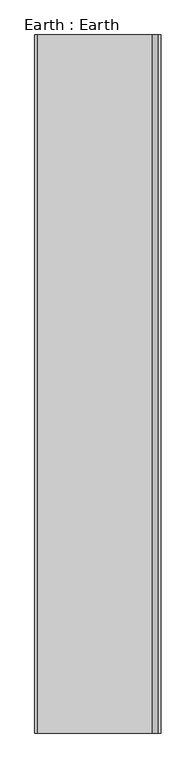
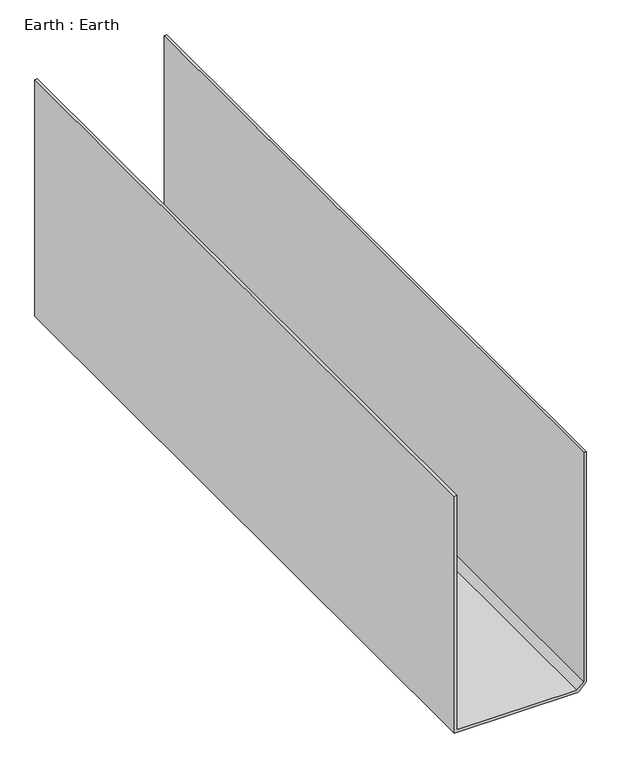
"""IFC4 building model written with IfcOpenShell, lengths in millimetres: proxy geometry, Earth : Earth."""

from ifc_helpers import new_model, si_unit, frame, origin, place, context, project, spatial, polyline, outline, extrude, source, transform, mapped, element, save


def earth_earth_d14d5190(model_context):
    return source(origin(), model_context, "Body", "SweptSolid", [
        extrude(outline(polyline([(32620.9902343, -10057.5706312), (32620.9902343, -9717.2148439), (32643.1028304, -9695.1022478), (33313.1445312, -9695.1022478), (33313.1445312, -9702.1022478), (32646.0023253, -9702.1022478), (32627.9902343, -9720.1143388), (32627.9902343, -10050.5706312), (33310.3609003, -10050.5706312), (33309.014262, -10057.5706312), (32620.9902343, -10057.5706312)])), frame((0.0, 7182.1531721, 0.0), z_axis=(0.0, 1.0, 0.0), x_axis=(0.0, 0.0, 1.0)), (0.0, 0.0, 1.0), 2000.0),
    ])


if __name__ == "__main__":
    model = new_model("IFC4")
    model_context = context("Model", 3, world=origin())
    ifc_project = project(units=[si_unit("LENGTHUNIT", "METRE", prefix="MILLI")], contexts=[model_context])
    site = spatial("IfcSite", under=ifc_project)
    building = spatial("IfcBuilding", under=site)
    placement = place(None, origin())
    earth_earth_shape = earth_earth_d14d5190(model_context)
    element("IfcBuildingElementProxy", 1, Name="Earth : Earth", ObjectType="Earth : Earth", at=placement, inside=building, context=model_context, shape_type="MappedRepresentation", body=[
        mapped(earth_earth_shape, transform((0.0, 0.0, 0.0), x_axis=(1.0, 0.0, 0.0), y_axis=(0.0, 1.0, 0.0), z_axis=(0.0, 0.0, 1.0))),
    ])
    save(model, "model.ifc")

# Revit data of these elements
# Type "Earth : Earth"
#   NameOverride = "Earth"
# Element 1 (IfcBuildingElementProxy, "Earth : Earth")
#   Materials on its faces: "WATERPROOF FIBER GLASS PLANTER LINER"
# Materials
#   "WATERPROOF FIBER GLASS PLANTER LINER": class "Unassigned", colour RGB 221 220 200, transparency 0, Cost = 0
